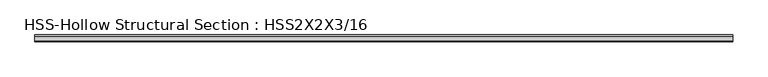
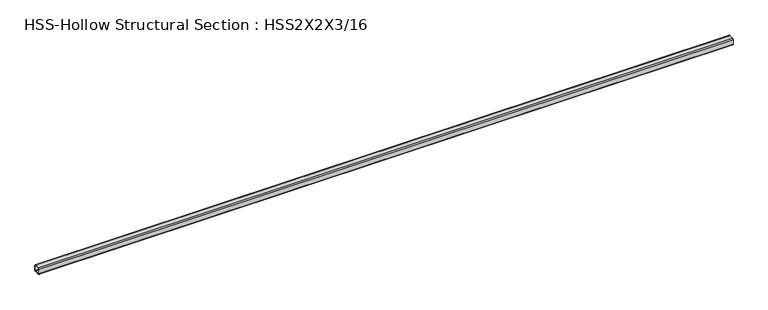
"""IFC4 building model written with IfcOpenShell, lengths in millimetres: beam geometry, HSS-Hollow Structural Section : HSS2X2X3/16."""

from ifc_helpers import new_model, si_unit, point, frame, frame_2d, origin, place, context, project, spatial, polyline, circle_curve, trimmed, segment, composite_curve, outline, extrude, source, transform, mapped, element, save


def hss_hollow_structural_section_hss2x2x3_16_2c82e856(model_context):
    return source(origin(), model_context, "Body", "SweptSolid", [
        extrude(outline(composite_curve([segment(polyline([(25.4, 16.5608), (25.4, -16.5608)]), True, "CONTINUOUS"), segment(trimmed(circle_curve(frame_2d((16.5608, -16.5608)), 8.8392), [point((25.4, -16.5608))], [point((16.5608, -25.4))], False, "CARTESIAN"), True, "CONTINUOUS"), segment(polyline([(16.5608, -25.4), (-16.5608, -25.4)]), True, "CONTINUOUS"), segment(trimmed(circle_curve(frame_2d((-16.5608, -16.5608)), 8.8392), [point((-16.5608, -25.4))], [point((-25.4, -16.5608))], False, "CARTESIAN"), True, "CONTINUOUS"), segment(polyline([(-25.4, -16.5608), (-25.4, 16.5608)]), True, "CONTINUOUS"), segment(trimmed(circle_curve(frame_2d((-16.5608, 16.5608)), 8.8392), [point((-25.4, 16.5608))], [point((-16.5608, 25.4))], False, "CARTESIAN"), True, "CONTINUOUS"), segment(polyline([(-16.5608, 25.4), (16.5608, 25.4)]), True, "CONTINUOUS"), segment(trimmed(circle_curve(frame_2d((16.5608, 16.5608)), 8.8392), [point((16.5608, 25.4))], [point((25.4, 16.5608))], False, "CARTESIAN"), True, "CONTINUOUS")], self_intersect=False), holes=[composite_curve([segment(trimmed(circle_curve(frame_2d((-16.5608, 16.5608)), 4.4196), [point((-16.5608, 20.9804))], [point((-20.9804, 16.5608))], True, "CARTESIAN"), True, "CONTINUOUS"), segment(polyline([(-20.9804, 16.5608), (-20.9804, -16.5608)]), True, "CONTINUOUS"), segment(trimmed(circle_curve(frame_2d((-16.5608, -16.5608)), 4.4196), [point((-20.9804, -16.5608))], [point((-16.5608, -20.9804))], True, "CARTESIAN"), True, "CONTINUOUS"), segment(polyline([(-16.5608, -20.9804), (16.5608, -20.9804)]), True, "CONTINUOUS"), segment(trimmed(circle_curve(frame_2d((16.5608, -16.5608)), 4.4196), [point((16.5608, -20.9804))], [point((20.9804, -16.5608))], True, "CARTESIAN"), True, "CONTINUOUS"), segment(polyline([(20.9804, -16.5608), (20.9804, 16.5608)]), True, "CONTINUOUS"), segment(trimmed(circle_curve(frame_2d((16.5608, 16.5608)), 4.4196), [point((20.9804, 16.5608))], [point((16.5608, 20.9804))], True, "CARTESIAN"), True, "CONTINUOUS"), segment(polyline([(16.5608, 20.9804), (-16.5608, 20.9804)]), True, "CONTINUOUS")], self_intersect=False)]), frame((4361.65625, 0.0, 0.0), z_axis=(1.0, 0.0, 0.0), x_axis=(0.0, 1.0, 0.0)), (0.0, 0.0, 1.0), 5127.625),
    ])


if __name__ == "__main__":
    model = new_model("IFC4")
    model_context = context("Model", 3, world=origin())
    ifc_project = project(units=[si_unit("LENGTHUNIT", "METRE", prefix="MILLI")], contexts=[model_context])
    site = spatial("IfcSite", under=ifc_project)
    building = spatial("IfcBuilding", under=site)
    placement = place(None, origin())
    hss_hollow_structural_section_hss2x2x3_16_shape = hss_hollow_structural_section_hss2x2x3_16_2c82e856(model_context)
    element("IfcBeam", 1, ObjectType="HSS-Hollow Structural Section : HSS2X2X3/16", at=placement, inside=building, context=model_context, shape_type="MappedRepresentation", body=[
        mapped(hss_hollow_structural_section_hss2x2x3_16_shape, transform((0.0, 0.0, 0.0), x_axis=(1.0, 0.0, 0.0), y_axis=(0.0, 1.0, 0.0), z_axis=(0.0, 0.0, 1.0))),
    ])
    save(model, "model.ifc")

# Revit data of these elements
# Type "HSS-Hollow Structural Section : HSS2X2X3/16"
#   Keynote = "M05121300.04"
#   Assembly Code = "B10"
#   Shape = "Square"
#   W = 4.3
#   Ht = 0' - 2"
#   Length [instance default] = 5' - 0"
#   b = 0' - 2"
#   kr = 0' - 0.348"
#   t = 0' - 0.174"
#   A = 0.00826389 SF
#   Structural Material [instance default] = Steel ASTM A500, Grade B, Rectangular and Square
# Element 1 (IfcBeam, "HSS-Hollow Structural Section : HSS2X2X3/16")
#   Materials on its faces: "Steel ASTM A500, Grade B, Rectangular and Square"
# Materials
#   "Steel ASTM A500, Grade B, Rectangular and Square": class "Metal", colour RGB 199 199 199, transparency 0, Description = "Carbon steel", Cost = 0
